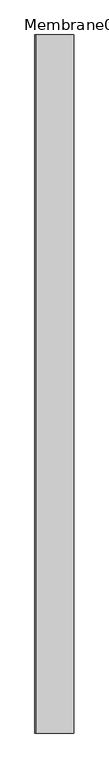
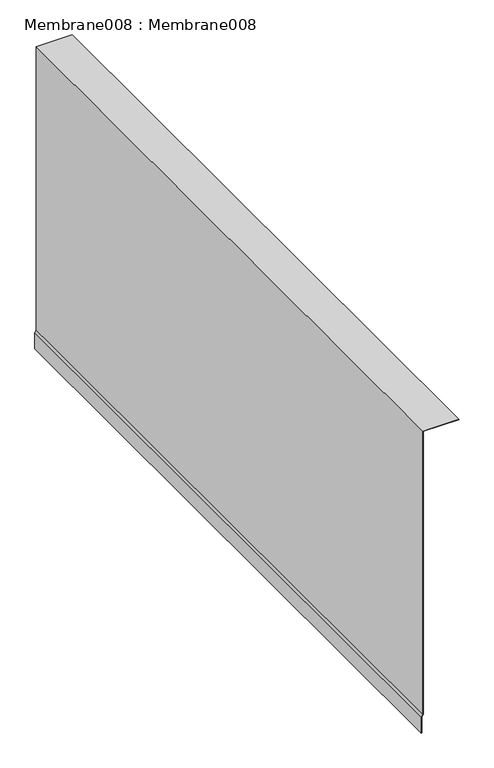
"""IFC4 building model written with IfcOpenShell, lengths in millimetres: proxy geometry, Membrane008 : Membrane008."""

from ifc_helpers import new_model, si_unit, frame, origin, place, context, project, spatial, polyline, outline, extrude, source, transform, mapped, element, save


def membrane008_membrane008_342d7b8d(model_context):
    return source(origin(), model_context, "Body", "SweptSolid", [
        extrude(outline(polyline([(33390.5106703, -9680.9523707), (33397.5184828, -9676.7926596), (34290.438014, -9676.7926596), (34290.438014, -9570.993191), (34291.938014, -9570.993191), (34291.938014, -9678.2926596), (33397.9301395, -9678.2926596), (33390.922327, -9682.4523707), (33340.7177015, -9682.4523707), (33340.7177015, -9680.9523707), (33390.5106703, -9680.9523707)])), frame((0.0, 7982.1529359, 0.0), z_axis=(0.0, 1.0, 0.0), x_axis=(0.0, 0.0, 1.0)), (0.0, 0.0, 1.0), 2000.0),
    ])


if __name__ == "__main__":
    model = new_model("IFC4")
    model_context = context("Model", 3, world=origin())
    ifc_project = project(units=[si_unit("LENGTHUNIT", "METRE", prefix="MILLI")], contexts=[model_context])
    site = spatial("IfcSite", under=ifc_project)
    building = spatial("IfcBuilding", under=site)
    placement = place(None, origin())
    membrane008_membrane008_shape = membrane008_membrane008_342d7b8d(model_context)
    element("IfcBuildingElementProxy", 1, Name="Membrane008 : Membrane008", ObjectType="Membrane008 : Membrane008", at=placement, inside=building, context=model_context, shape_type="MappedRepresentation", body=[
        mapped(membrane008_membrane008_shape, transform((0.0, 0.0, 0.0), x_axis=(1.0, 0.0, 0.0), y_axis=(0.0, 1.0, 0.0), z_axis=(0.0, 0.0, 1.0))),
    ])
    save(model, "model.ifc")

# Revit data of these elements
# Type "Membrane008 : Membrane008"
#   NameOverride = "Membrane008"
# Element 1 (IfcBuildingElementProxy, "Membrane008 : Membrane008")
#   Materials on its faces: "2 LAYERS NO. 30 ASTM D226 ASPHALT SATURATED ORGANIC FELT"
# Materials
#   "2 LAYERS NO. 30 ASTM D226 ASPHALT SATURATED ORGANIC FELT": class "Unassigned", colour RGB 46 171 0, transparency 0
